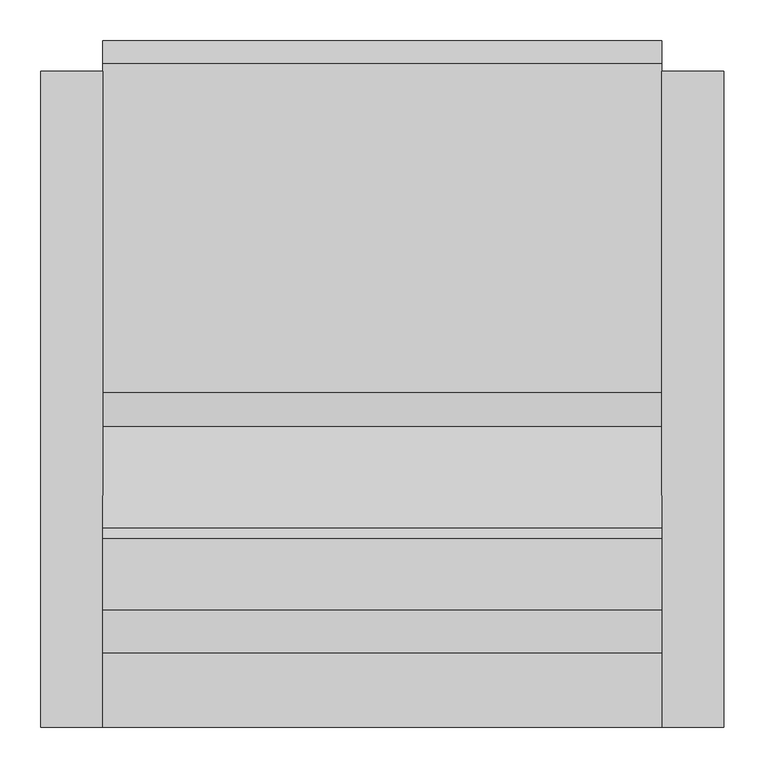
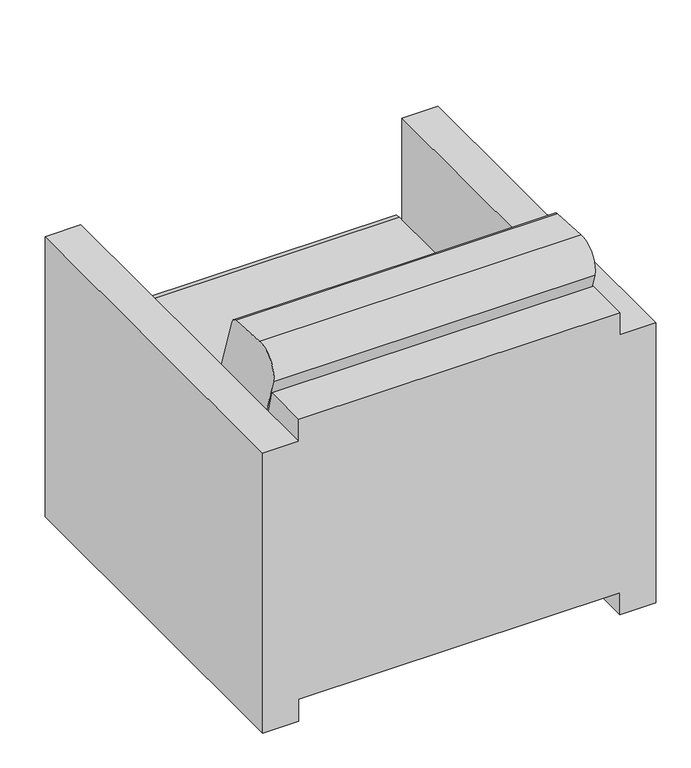
"""IFC4 building model written with IfcOpenShell, lengths in millimetres: furniture geometry, Chair, Lounge-NON-COLLECTUS : -."""

from ifc_helpers import new_model, si_unit, point, frame, frame_2d, origin, place, context, project, spatial, polyline, circle_curve, trimmed, segment, composite_curve, outline, extrude, faceted_brep, source, transform, mapped, element, save


def furniture_4144d577(model_context):
    return source(origin(), model_context, "Body", "SolidModel", [
        faceted_brep([(76.2, -35.4707031, 0.0), (76.2, -35.4707031, 50.0), (76.2, -839.99832, 50.0), (76.2, -839.99832, 0.0), (76.2, -728.8741489, 630.998418), (76.2, -629.6925584, 250.0), (76.2, -35.4707031, 250.0), (76.2, -35.4707031, 630.998418), (0.0, -839.99832, 0.0), (0.0, -839.99832, 630.998418), (0.0, -35.4707031, 630.998418), (0.0, -35.4707031, 0.0), (761.798324, -839.99832, 50.0), (761.798324, -839.99832, 0.0), (837.998324, -839.99832, 0.0), (837.998324, -839.99832, 630.998418), (761.798324, -839.99832, 630.998418), (761.798324, -839.99832, 680.998418), (76.2, -839.99832, 680.998418), (76.2, -839.99832, 630.998418), (761.798324, -35.4707031, 250.0), (761.798324, -35.4707031, 630.998418), (837.998324, -35.4707031, 630.998418), (837.998324, -35.4707031, 0.0), (761.798324, -35.4707031, 0.0), (761.798324, -35.4707031, 50.0), (761.798324, -728.8741489, 630.998418), (761.798324, -741.8901597, 680.998418), (76.2, -741.8901597, 680.998418), (761.798324, -629.6925584, 250.0)], [[[0, 1, 2, 3]], [[4, 5, 6, 7]], [[8, 9, 10, 11]], [[8, 3, 2, 12, 13, 14, 15, 16, 17, 18, 19, 9]], [[9, 19, 4, 7, 10]], [[10, 7, 6, 20, 21, 22, 23, 24, 25, 1, 0, 11]], [[3, 8, 11, 0]], [[17, 16, 26, 27]], [[28, 4, 19, 18]], [[29, 20, 6, 5]], [[25, 12, 2, 1]], [[27, 28, 18, 17]], [[5, 4, 28, 27, 26, 29]], [[14, 23, 22, 15]], [[13, 12, 25, 24]], [[20, 29, 26, 21]], [[22, 21, 26, 16, 15]], [[14, 13, 24, 23]]]),
        extrude(outline(composite_curve([segment(trimmed(circle_curve(frame_2d((-699.4337939, 720.1804436)), 49.2227188), [point((-747.4296917, 709.2593701))], [point((-696.0604701, 769.2874364))], False, "CARTESIAN"), True, "CONTINUOUS"), segment(polyline([(-696.0604701, 769.2874364), (-609.080933, 763.3125207)]), True, "CONTINUOUS"), segment(trimmed(circle_curve(frame_2d((-610.1450412, 747.8218184)), 15.5272079), [point((-609.080933, 763.3125207))], [point((-595.2985323, 752.3688349))], False, "CARTESIAN"), True, "CONTINUOUS"), segment(polyline([(-595.2985323, 752.3688349), (-471.2304221, 374.9461126)]), True, "CONTINUOUS"), segment(trimmed(circle_curve(frame_2d((-428.8095819, 354.8200478)), 46.9530208), [point((-471.2304221, 374.9461126))], [point((-428.8095819, 401.7730686))], False, "CARTESIAN"), True, "CONTINUOUS"), segment(polyline([(-428.8095819, 401.7730686), (-25.8559684, 401.7730686)]), True, "CONTINUOUS"), segment(trimmed(circle_curve(frame_2d((-25.8559684, 373.8331399)), 27.9399287), [point((-25.8559684, 401.7730686))], [point((-0.5447429, 362.001763))], False, "CARTESIAN"), True, "CONTINUOUS"), segment(polyline([(-0.5447429, 362.001763), (-18.011651, 270.6587956)]), True, "CONTINUOUS"), segment(trimmed(circle_curve(frame_2d((-42.6318449, 275.0)), 25.0), [point((-18.011651, 270.6587956))], [point((-42.6318449, 250.0))], False, "CARTESIAN"), True, "CONTINUOUS"), segment(polyline([(-42.6318449, 250.0), (-602.5633793, 250.0), (-747.4296917, 709.2593701)]), True, "CONTINUOUS")], self_intersect=False)), frame((76.2, 0.0, 0.0), z_axis=(1.0, 0.0, 0.0), x_axis=(0.0, 1.0, 0.0)), (0.0, 0.0, 1.0), 685.598324),
    ])


if __name__ == "__main__":
    model = new_model("IFC4")
    model_context = context("Model", 3, world=origin())
    ifc_project = project(units=[si_unit("LENGTHUNIT", "METRE", prefix="MILLI")], contexts=[model_context])
    site = spatial("IfcSite", under=ifc_project)
    building = spatial("IfcBuilding", under=site)
    placement = place(None, origin())
    furniture_shape = furniture_4144d577(model_context)
    element("IfcFurniture", 1, ObjectType="Chair, Lounge-NON-COLLECTUS : -", at=placement, inside=building, context=model_context, shape_type="MappedRepresentation", body=[
        mapped(furniture_shape, transform((0.0, 0.0, 0.0), x_axis=(1.0, 0.0, 0.0), y_axis=(0.0, 1.0, 0.0), z_axis=(0.0, 0.0, 1.0))),
    ])
    save(model, "model.ifc")

# Revit data of these elements
# Type "Chair, Lounge-NON-COLLECTUS : -"
#   External ID [instance default] = ""
#   projection = 35.52 mm
#   Width = 837.998 mm
#   Height = 790.998 mm
#   Depth = 839.998 mm
#   Arm Width = 76.2 mm
#   Frame = White
#   Cushion = White
#   Default Elevation = 0
# Element 1 (IfcFurniture, "Chair, Lounge-NON-COLLECTUS : -")
#   Materials on its faces: "White"
# Materials
#   "White": class "Generic", colour RGB 255 255 255, transparency 0, Cost = 0
